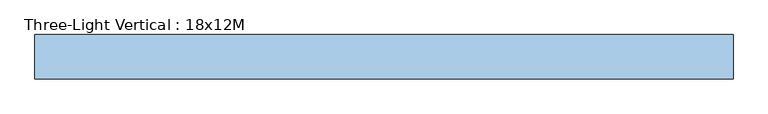
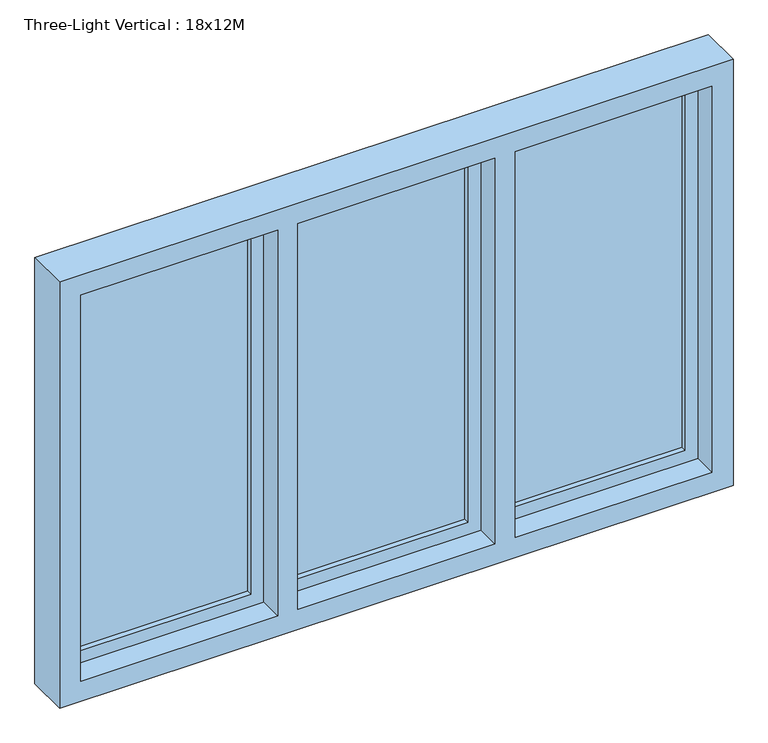
"""IFC4 building model written with IfcOpenShell, lengths in millimetres: window geometry, Three-Light Vertical : 18x12M."""

from ifc_helpers import new_model, si_unit, frame, origin, place, context, project, spatial, polyline, outline, extrude, faceted_brep, source, transform, mapped, element, save


def three_light_vertical_18x12m_b3fc569e(model_context):
    return source(origin(), model_context, "Body", "SolidModel", [
        extrude(outline(polyline([(1970.0, -924.0), (842.0, -924.0), (842.0, -364.6666667), (1970.0, -364.6666667), (1970.0, -924.0)]), holes=[polyline([(1920.0, -414.6666667), (892.0, -414.6666667), (892.0, -874.0), (1920.0, -874.0), (1920.0, -414.6666667)])]), frame((0.0, 134.0, 0.0), z_axis=(0.0, 1.0, 0.0), x_axis=(0.0, 0.0, 1.0)), (0.0, 0.0, 1.0), 50.0),
        extrude(outline(polyline([(1970.0, -339.6666667), (842.0, -339.6666667), (842.0, 219.6666667), (1970.0, 219.6666667), (1970.0, -339.6666667)]), holes=[polyline([(1920.0, 169.6666667), (892.0, 169.6666667), (892.0, -289.6666667), (1920.0, -289.6666667), (1920.0, 169.6666667)])]), frame((0.0, 134.0, 0.0), z_axis=(0.0, 1.0, 0.0), x_axis=(0.0, 0.0, 1.0)), (0.0, 0.0, 1.0), 50.0),
        extrude(outline(polyline([(1970.0, 244.6666667), (842.0, 244.6666667), (842.0, 804.0), (1970.0, 804.0), (1970.0, 244.6666667)]), holes=[polyline([(1920.0, 754.0), (892.0, 754.0), (892.0, 294.6666667), (1920.0, 294.6666667), (1920.0, 754.0)])]), frame((0.0, 134.0, 0.0), z_axis=(0.0, 1.0, 0.0), x_axis=(0.0, 0.0, 1.0)), (0.0, 0.0, 1.0), 50.0),
        faceted_brep([(-966.0, 184.0, 800.0), (846.0, 184.0, 800.0), (846.0, 69.0, 800.0), (-966.0, 69.0, 800.0), (846.0, 184.0, 2012.0), (846.0, 69.0, 2012.0), (-966.0, 184.0, 2012.0), (804.0, 184.0, 842.0), (804.0, 184.0, 1970.0), (244.6666667, 184.0, 1970.0), (244.6666667, 184.0, 842.0), (-924.0, 184.0, 1970.0), (-924.0, 184.0, 842.0), (-364.6666667, 184.0, 842.0), (-364.6666667, 184.0, 1970.0), (219.6666667, 184.0, 1970.0), (-339.6666667, 184.0, 1970.0), (-339.6666667, 184.0, 842.0), (219.6666667, 184.0, 842.0), (-966.0, 69.0, 2012.0), (789.0, 69.0, 1955.0), (789.0, 69.0, 857.0), (259.6666667, 69.0, 857.0), (259.6666667, 69.0, 1955.0), (204.6666667, 69.0, 857.0), (-324.6666667, 69.0, 857.0), (-324.6666667, 69.0, 1955.0), (204.6666667, 69.0, 1955.0), (-909.0, 69.0, 857.0), (-909.0, 69.0, 1955.0), (-379.6666667, 69.0, 1955.0), (-379.6666667, 69.0, 857.0), (789.0, 134.0, 857.0), (259.6666667, 134.0, 857.0), (-909.0, 134.0, 857.0), (-379.6666667, 134.0, 857.0), (204.6666667, 134.0, 857.0), (-324.6666667, 134.0, 857.0), (789.0, 134.0, 1955.0), (804.0, 134.0, 1970.0), (804.0, 134.0, 842.0), (244.6666667, 134.0, 842.0), (244.6666667, 134.0, 1970.0), (259.6666667, 134.0, 1955.0), (-924.0, 134.0, 842.0), (-924.0, 134.0, 1970.0), (-364.6666667, 134.0, 1970.0), (-364.6666667, 134.0, 842.0), (-909.0, 134.0, 1955.0), (-379.6666667, 134.0, 1955.0), (219.6666667, 134.0, 1970.0), (219.6666667, 134.0, 842.0), (-339.6666667, 134.0, 842.0), (-339.6666667, 134.0, 1970.0), (204.6666667, 134.0, 1955.0), (-324.6666667, 134.0, 1955.0)], [[[0, 1, 2, 3]], [[2, 1, 4, 5]], [[4, 1, 0, 6], [7, 8, 9, 10], [11, 12, 13, 14], [15, 16, 17, 18]], [[2, 5, 19, 3], [20, 21, 22, 23], [24, 25, 26, 27], [28, 29, 30, 31]], [[21, 32, 33, 22]], [[34, 28, 31, 35]], [[24, 36, 37, 25]], [[32, 21, 20, 38]], [[39, 40, 41, 42], [32, 38, 43, 33]], [[44, 45, 46, 47], [48, 34, 35, 49]], [[50, 51, 52, 53], [36, 54, 55, 37]], [[52, 51, 18, 17]], [[40, 7, 10, 41]], [[12, 44, 47, 13]], [[7, 40, 39, 8]], [[19, 6, 0, 3]], [[48, 29, 28, 34]], [[11, 45, 44, 12]], [[10, 9, 42, 41]], [[23, 22, 33, 43]], [[24, 27, 54, 36]], [[15, 18, 51, 50]], [[17, 16, 53, 52]], [[26, 25, 37, 55]], [[31, 30, 49, 35]], [[14, 13, 47, 46]], [[19, 5, 4, 6]], [[38, 20, 23, 43]], [[29, 48, 49, 30]], [[54, 27, 26, 55]], [[8, 39, 42, 9]], [[15, 50, 53, 16]], [[46, 45, 11, 14]]]),
        extrude(outline(polyline([(-289.6666667, 170.0), (169.6666667, 170.0), (169.6666667, 148.0), (-289.6666667, 148.0), (-289.6666667, 170.0)])), frame((0.0, 0.0, 892.0), z_axis=(0.0, 0.0, 1.0), x_axis=(1.0, 0.0, 0.0)), (0.0, 0.0, 1.0), 1028.0),
        extrude(outline(polyline([(-874.0, 170.0), (-414.6666667, 170.0), (-414.6666667, 148.0), (-874.0, 148.0), (-874.0, 170.0)])), frame((0.0, 0.0, 892.0), z_axis=(0.0, 0.0, 1.0), x_axis=(1.0, 0.0, 0.0)), (0.0, 0.0, 1.0), 1028.0),
        extrude(outline(polyline([(294.6666667, 170.0), (754.0, 170.0), (754.0, 148.0), (294.6666667, 148.0), (294.6666667, 170.0)])), frame((0.0, 0.0, 892.0), z_axis=(0.0, 0.0, 1.0), x_axis=(1.0, 0.0, 0.0)), (0.0, 0.0, 1.0), 1028.0),
    ])


if __name__ == "__main__":
    model = new_model("IFC4")
    model_context = context("Model", 3, world=origin())
    ifc_project = project(units=[si_unit("LENGTHUNIT", "METRE", prefix="MILLI")], contexts=[model_context])
    site = spatial("IfcSite", under=ifc_project)
    building = spatial("IfcBuilding", under=site)
    placement = place(None, origin())
    three_light_vertical_18x12m_shape = three_light_vertical_18x12m_b3fc569e(model_context)
    element("IfcWindow", 1, ObjectType="Three-Light Vertical : 18x12M", at=placement, inside=building, context=model_context, shape_type="MappedRepresentation", body=[
        mapped(three_light_vertical_18x12m_shape, transform((0.0, 0.0, 0.0), x_axis=(1.0, 0.0, 0.0), y_axis=(0.0, 1.0, 0.0), z_axis=(0.0, 0.0, 1.0))),
    ])
    save(model, "model.ifc")

# Revit data of these elements
# Type "Three-Light Vertical : 18x12M"
#   Type Mark = "50"
#   Creator Organization [instance default] = "© Danish Educational Content"
#   Creator Name [instance default] = "© Erik Falck Jørgensen"
#   Creator Build [instance default] = "2017.0801.0"
#   Analytic Construction = "<None>"
#   length#6 = -36 mm
#   length#5 = -14 mm
#   length#4 = 120 mm
#   length#3 = 29.5 mm
#   length#2 = 57 mm
#   length#1 = 0 mm
#   Seal Width = 12 mm
#   Rough Width = 1812 mm
#   Rough Height = 1212 mm
#   Rebate Depth = 50 mm
#   Transom Width = 55 mm
#   Rabbet Width = 15 mm
#   Rabbet Depth = 50 mm
#   Height = 1188 mm
#   Glass Thickness = 22 mm
#   Frame Width = 50 mm
#   Frame Depth = 50 mm
#   Exterior Direction [instance default] = 0.00°
#   Case Depth = 115 mm
#   Case Width = 45 mm
#   Default Sill Height = 800 mm
#   Width = 1788 mm
#   Sealing = no
#   Hinging = yes
#   Wall Closure = 1
#   Above Cutplane [instance default] = no
#   Glass = none
#   Case/Transom = none
#   Frame/Mullion = none
#   Assembly Code = ""
# Element 1 (IfcWindow, "Three-Light Vertical : 18x12M")
#   Materials on its faces: "Default Frame/Mullion (Interior/Exterior)", "Glass"
# Materials
#   "Default Frame/Mullion (Interior/Exterior)": class "Generic", colour RGB 205 205 205, transparency 0, Description = "Udefineret karm/ramme materiale", Cost = 0
#   "Glass": class "Glass", colour RGB 180 200 255, transparency 0.75, Description = "Generisk glas", Cost = 0
